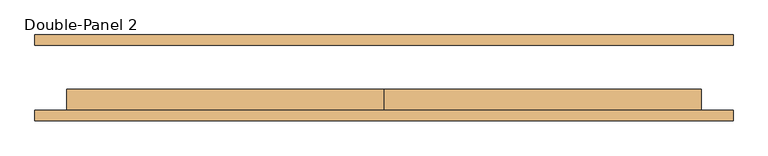
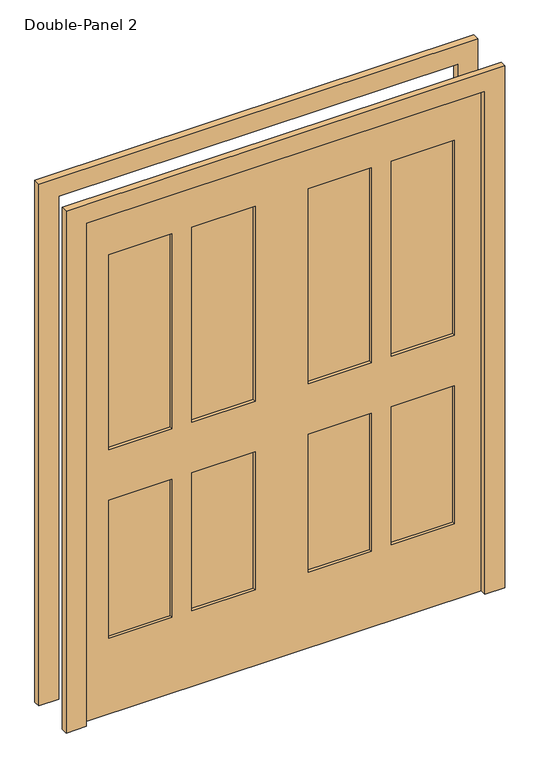
"""IFC4 building model written with IfcOpenShell, lengths in millimetres: door geometry, Double-Panel 2."""

from ifc_helpers import new_model, si_unit, frame, origin, place, context, project, spatial, polyline, outline, extrude, source, transform, mapped, element, save


def double_panel_2_e6a16e79(model_context):
    return source(origin(), model_context, "Body", "SweptSolid", [
        extrude(outline(polyline([(2108.2, -838.2), (0.0, -838.2), (0.0, -762.0), (2032.0, -762.0), (2032.0, 762.0), (0.0, 762.0), (0.0, 838.2), (2108.2, 838.2), (2108.2, -838.2)])), frame((0.0, -103.1875, 0.0), z_axis=(0.0, 1.0, 0.0), x_axis=(0.0, 0.0, 1.0)), (0.0, 0.0, 1.0), 25.4),
        extrude(outline(polyline([(419.1, -65.0875), (419.1, -39.6875), (660.4, -39.6875), (660.4, -65.0875), (419.1, -65.0875)])), frame((0.0, 0.0, 1066.8), z_axis=(0.0, 0.0, 1.0), x_axis=(1.0, 0.0, 0.0)), (0.0, 0.0, 1.0), 787.4),
        extrude(outline(polyline([(101.6, -65.0875), (101.6, -39.6875), (342.9, -39.6875), (342.9, -65.0875), (101.6, -65.0875)])), frame((0.0, 0.0, 1066.8), z_axis=(0.0, 0.0, 1.0), x_axis=(1.0, 0.0, 0.0)), (0.0, 0.0, 1.0), 787.4),
        extrude(outline(polyline([(419.1, -65.0875), (419.1, -39.6875), (660.4, -39.6875), (660.4, -65.0875), (419.1, -65.0875)])), frame((0.0, 0.0, 304.8), z_axis=(0.0, 0.0, 1.0), x_axis=(1.0, 0.0, 0.0)), (0.0, 0.0, 1.0), 558.8),
        extrude(outline(polyline([(101.6, -65.0875), (101.6, -39.6875), (342.9, -39.6875), (342.9, -65.0875), (101.6, -65.0875)])), frame((0.0, 0.0, 304.8), z_axis=(0.0, 0.0, 1.0), x_axis=(1.0, 0.0, 0.0)), (0.0, 0.0, 1.0), 558.8),
        extrude(outline(polyline([(-342.9, -65.0875), (-342.9, -39.6875), (-101.6, -39.6875), (-101.6, -65.0875), (-342.9, -65.0875)])), frame((0.0, 0.0, 1066.8), z_axis=(0.0, 0.0, 1.0), x_axis=(1.0, 0.0, 0.0)), (0.0, 0.0, 1.0), 787.4),
        extrude(outline(polyline([(-660.4, -65.0875), (-660.4, -39.6875), (-419.1, -39.6875), (-419.1, -65.0875), (-660.4, -65.0875)])), frame((0.0, 0.0, 1066.8), z_axis=(0.0, 0.0, 1.0), x_axis=(1.0, 0.0, 0.0)), (0.0, 0.0, 1.0), 787.4),
        extrude(outline(polyline([(-342.9, -65.0875), (-342.9, -39.6875), (-101.6, -39.6875), (-101.6, -65.0875), (-342.9, -65.0875)])), frame((0.0, 0.0, 304.8), z_axis=(0.0, 0.0, 1.0), x_axis=(1.0, 0.0, 0.0)), (0.0, 0.0, 1.0), 558.8),
        extrude(outline(polyline([(-660.4, -65.0875), (-660.4, -39.6875), (-419.1, -39.6875), (-419.1, -65.0875), (-660.4, -65.0875)])), frame((0.0, 0.0, 304.8), z_axis=(0.0, 0.0, 1.0), x_axis=(1.0, 0.0, 0.0)), (0.0, 0.0, 1.0), 558.8),
        extrude(outline(polyline([(2032.0, 0.0), (2032.0, -762.0), (0.0, -762.0), (0.0, 0.0), (0.0, 762.0), (2032.0, 762.0), (2032.0, 0.0)]), holes=[polyline([(1854.2, 419.1), (1854.2, 660.4), (1066.8, 660.4), (1066.8, 419.1), (1854.2, 419.1)]), polyline([(1854.2, 101.6), (1854.2, 342.9), (1066.8, 342.9), (1066.8, 101.6), (1854.2, 101.6)]), polyline([(863.6, 419.1), (863.6, 660.4), (304.8, 660.4), (304.8, 419.1), (863.6, 419.1)]), polyline([(863.6, 101.6), (863.6, 342.9), (304.8, 342.9), (304.8, 101.6), (863.6, 101.6)]), polyline([(1066.8, -342.9), (1854.2, -342.9), (1854.2, -101.6), (1066.8, -101.6), (1066.8, -342.9)]), polyline([(1854.2, -660.4), (1854.2, -419.1), (1066.8, -419.1), (1066.8, -660.4), (1854.2, -660.4)]), polyline([(863.6, -342.9), (863.6, -101.6), (304.8, -101.6), (304.8, -342.9), (863.6, -342.9)]), polyline([(863.6, -660.4), (863.6, -419.1), (304.8, -419.1), (304.8, -660.4), (863.6, -660.4)])]), frame((0.0, -77.7875, 0.0), z_axis=(0.0, 1.0, 0.0), x_axis=(0.0, 0.0, 1.0)), (0.0, 0.0, 1.0), 50.8),
        extrude(outline(polyline([(2032.0, -762.0), (2032.0, 762.0), (0.0, 762.0), (0.0, 838.2), (2108.2, 838.2), (2108.2, -838.2), (0.0, -838.2), (0.0, -762.0), (2032.0, -762.0)])), frame((0.0, 77.7875, 0.0), z_axis=(0.0, 1.0, 0.0), x_axis=(0.0, 0.0, 1.0)), (0.0, 0.0, 1.0), 25.4),
    ])


if __name__ == "__main__":
    model = new_model("IFC4")
    model_context = context("Model", 3, world=origin())
    ifc_project = project(units=[si_unit("LENGTHUNIT", "METRE", prefix="MILLI")], contexts=[model_context])
    site = spatial("IfcSite", under=ifc_project)
    building = spatial("IfcBuilding", under=site)
    placement = place(None, origin())
    double_panel_2_shape = double_panel_2_e6a16e79(model_context)
    element("IfcDoor", 1, ObjectType="Double-Panel 2 : 60\" x 80\"  White", at=placement, inside=building, context=model_context, shape_type="MappedRepresentation", body=[
        mapped(double_panel_2_shape, transform((0.0, 0.0, 0.0), x_axis=(1.0, 0.0, 0.0), y_axis=(0.0, 1.0, 0.0), z_axis=(0.0, 0.0, 1.0))),
    ])
    save(model, "model.ifc")

# Revit data of these elements
# Type "Double-Panel 2 : 60\" x 80\"  White"
#   Type Mark = "85"
#   COBie.Type.CreatedBy = "doug.wood@us.ibm.com"
#   COBie.Type.CreatedOn = "2016-04-14T02:07:24"
#   COBie.Type.Name = "Doors_Double-Panel 2_60\" x 80\"  White_85"
#   COBie.Type.Category = "23-30 10 00 : Doors"
#   COBie.Type.Description = "Double-Panel 2_60\" x 80\"  White"
#   COBie.Type.Manufacturer = ""
#   COBie.Type.ModelNumber = ""
#   Construction Type Id = "MDOOR"
#   Assembly Code = "C1020"
#   Analytic Construction = "Metal"
#   COBie.Type.ReplacementCost = 0
#   Thickness = 0' - 2"
#   Heat Transfer Coefficient (U) = 3.7021 W/(m²·K)
#   Height = 6' - 8"
#   Trim Projection Ext = 0' - 1"
#   Trim Projection Int = 0' - 1"
#   Trim Width = 0' - 3"
#   Width = 5' - 0"
#   COBie.Type = no
#   Door Material = Door - Panel
#   Frame Material = Trim - White
#   Visual Light Transmittance = 0
#   Solar Heat Gain Coefficient = 0
#   Function = (empty or 0)
#   Wall Closure = (empty or 0)
# Element 1 (IfcDoor, "Double-Panel 2 : 60\" x 80\"  White")
#   Materials on its faces: "Door - Panel", "Trim - White"
# Materials
#   "Door - Panel": class "Wood", colour RGB 255 255 255, transparency 0, Cost = 0
#   "Trim - White": class "Wood", colour RGB 255 255 255, transparency 0, Cost = 0
